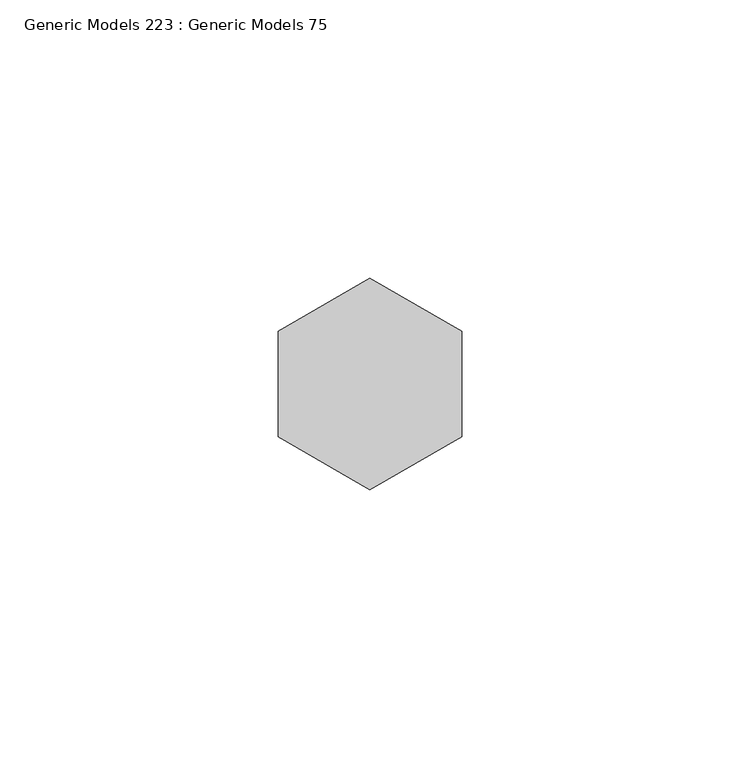
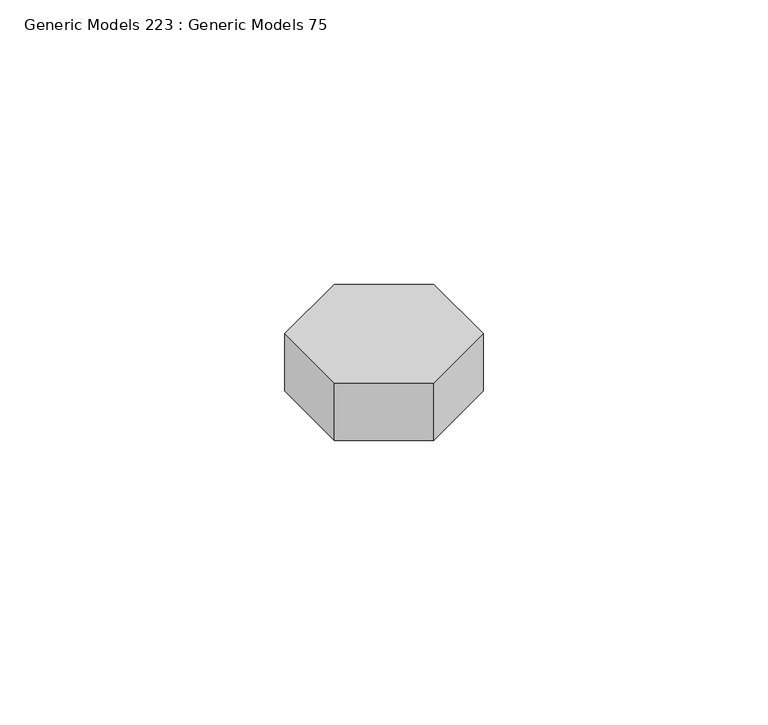
"""IFC4 building model written with IfcOpenShell, lengths in millimetres: proxy geometry, Generic Models 223 : Generic Models 75."""

from ifc_helpers import new_model, si_unit, frame, origin, place, context, project, spatial, polyline, outline, extrude, source, transform, mapped, element, save


def generic_models_223_generic_models_75_c2a9037b(model_context):
    return source(origin(), model_context, "Body", "SweptSolid", [
        extrude(outline(polyline([(31991.9073871, 30887.1007369), (31975.4096032, 30877.5757369), (31958.9118192, 30887.1007369), (31958.9118192, 30906.1507369), (31975.4096032, 30915.6757369), (31991.9073871, 30906.1507369), (31991.9073871, 30887.1007369)])), frame((0.0, 0.0, 266422.1875), z_axis=(0.0, 0.0, 1.0), x_axis=(1.0, 0.0, 0.0)), (0.0, 0.0, 1.0), 13.49375),
    ])


if __name__ == "__main__":
    model = new_model("IFC4")
    model_context = context("Model", 3, world=origin())
    ifc_project = project(units=[si_unit("LENGTHUNIT", "METRE", prefix="MILLI")], contexts=[model_context])
    site = spatial("IfcSite", under=ifc_project)
    building = spatial("IfcBuilding", under=site)
    placement = place(None, origin())
    generic_models_223_generic_models_75_shape = generic_models_223_generic_models_75_c2a9037b(model_context)
    element("IfcBuildingElementProxy", 1, Name="Generic Models 223 : Generic Models 75", ObjectType="Generic Models 223 : Generic Models 75", at=placement, inside=building, context=model_context, shape_type="MappedRepresentation", body=[
        mapped(generic_models_223_generic_models_75_shape, transform((0.0, 0.0, 0.0), x_axis=(1.0, 0.0, 0.0), y_axis=(0.0, 1.0, 0.0), z_axis=(0.0, 0.0, 1.0))),
    ])
    save(model, "model.ifc")

# Revit data of these elements
# Element 1 (IfcBuildingElementProxy, "Generic Models 223 : Generic Models 75")
#   Materials on its faces: "5/8\" DIA. EPOXY ANCHOR BOLTS"
# Materials
#   "5/8\" DIA. EPOXY ANCHOR BOLTS": class "Metal", colour RGB 199 199 199, transparency 0, Description = "Carbon steel", Cost = 0
